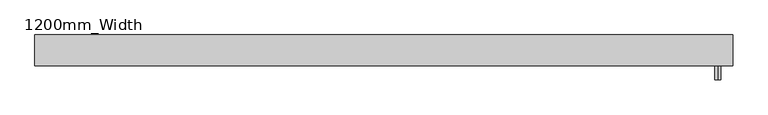
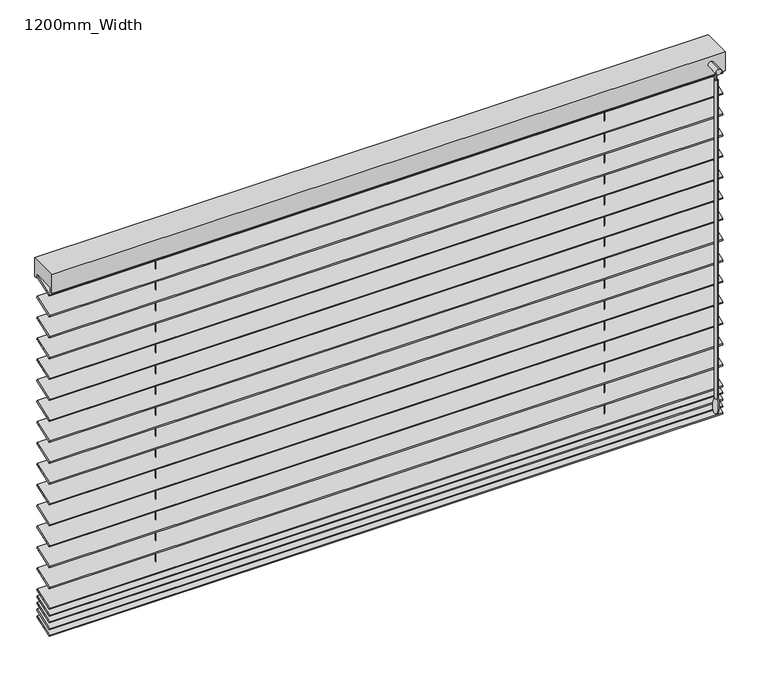
"""IFC4 building model written with IfcOpenShell, lengths in millimetres: proxy geometry, Specialty_Equipment_Venetian_Blind_Half_Down : 1200mm_Width."""

from ifc_helpers import new_model, si_unit, point, frame, frame_2d, origin, place, context, project, spatial, polyline, circle_curve, ellipse_curve, trimmed, segment, composite_curve, outline, extrude, source, transform, mapped, element, save
from ifc_brep_helpers import plane_surface, cylinder_surface, revolved_surface, advanced_brep


def proxy_1200mm_width_55fef7d2(model_context):
    return source(origin(), model_context, "Body", "SolidModel", [
        extrude(outline(polyline([(0.0, -40.0), (0.0, 0.0), (1180.0, 0.0), (1180.0, -40.0), (0.0, -40.0)])), frame((-439.5079376, 65.0532351, 1447.7279746), z_axis=(0.0, -0.3420201433256684, 0.9396926207859085), x_axis=(1.0, 0.0, 0.0)), (0.0, 0.0, 1.0), 3.0625345),
        extrude(outline(polyline([(0.0, -40.0), (0.0, 0.0), (1180.0, 0.0), (1180.0, -40.0), (0.0, -40.0)])), frame((-439.5079376, 65.0532351, 1459.9116214), z_axis=(0.0, -0.3420201433256684, 0.9396926207859085), x_axis=(1.0, 0.0, 0.0)), (0.0, 0.0, 1.0), 3.0625345),
        extrude(outline(polyline([(0.0, -40.0), (0.0, 0.0), (1180.0, 0.0), (1180.0, -40.0), (0.0, -40.0)])), frame((-439.5079376, 65.0532351, 1472.7202682), z_axis=(0.0, -0.3420201433256684, 0.9396926207859085), x_axis=(1.0, 0.0, 0.0)), (0.0, 0.0, 1.0), 3.0625345),
        extrude(outline(polyline([(0.0, -40.0), (0.0, 0.0), (1180.0, 0.0), (1180.0, -40.0), (0.0, -40.0)])), frame((-439.5079376, 65.0532351, 1484.903915), z_axis=(0.0, -0.3420201433256684, 0.9396926207859085), x_axis=(1.0, 0.0, 0.0)), (0.0, 0.0, 1.0), 3.0625345),
        extrude(outline(polyline([(0.0, -40.0), (0.0, 0.0), (1180.0, 0.0), (1180.0, -40.0), (0.0, -40.0)])), frame((-439.5079376, 65.0532351, 2040.2125618), z_axis=(0.0, -0.3420201433256684, 0.9396926207859085), x_axis=(1.0, 0.0, 0.0)), (0.0, 0.0, 1.0), 3.0625345),
        extrude(outline(polyline([(0.0, -40.0), (0.0, 0.0), (1180.0, 0.0), (1180.0, -40.0), (0.0, -40.0)])), frame((-439.5079376, 65.0532351, 2001.4625618), z_axis=(0.0, -0.3420201433256684, 0.9396926207859085), x_axis=(1.0, 0.0, 0.0)), (0.0, 0.0, 1.0), 3.0625345),
        extrude(outline(polyline([(0.0, -40.0), (0.0, 0.0), (1180.0, 0.0), (1180.0, -40.0), (0.0, -40.0)])), frame((-439.5079376, 65.0532351, 1962.7125618), z_axis=(0.0, -0.3420201433256684, 0.9396926207859085), x_axis=(1.0, 0.0, 0.0)), (0.0, 0.0, 1.0), 3.0625345),
        extrude(outline(polyline([(0.0, -40.0), (0.0, 0.0), (1180.0, 0.0), (1180.0, -40.0), (0.0, -40.0)])), frame((-439.5079376, 65.0532351, 1923.9625618), z_axis=(0.0, -0.3420201433256684, 0.9396926207859085), x_axis=(1.0, 0.0, 0.0)), (0.0, 0.0, 1.0), 3.0625345),
        extrude(outline(polyline([(0.0, -40.0), (0.0, 0.0), (1180.0, 0.0), (1180.0, -40.0), (0.0, -40.0)])), frame((-439.5079376, 65.0532351, 1885.2125618), z_axis=(0.0, -0.3420201433256684, 0.9396926207859085), x_axis=(1.0, 0.0, 0.0)), (0.0, 0.0, 1.0), 3.0625345),
        extrude(outline(polyline([(0.0, -40.0), (0.0, 0.0), (1180.0, 0.0), (1180.0, -40.0), (0.0, -40.0)])), frame((-439.5079376, 65.0532351, 1846.4625618), z_axis=(0.0, -0.3420201433256684, 0.9396926207859085), x_axis=(1.0, 0.0, 0.0)), (0.0, 0.0, 1.0), 3.0625345),
        extrude(outline(polyline([(0.0, -40.0), (0.0, 0.0), (1180.0, 0.0), (1180.0, -40.0), (0.0, -40.0)])), frame((-439.5079376, 65.0532351, 1807.7125618), z_axis=(0.0, -0.3420201433256684, 0.9396926207859085), x_axis=(1.0, 0.0, 0.0)), (0.0, 0.0, 1.0), 3.0625345),
        extrude(outline(polyline([(0.0, -40.0), (0.0, 0.0), (1180.0, 0.0), (1180.0, -40.0), (0.0, -40.0)])), frame((-439.5079376, 65.0532351, 1768.9625618), z_axis=(0.0, -0.3420201433256684, 0.9396926207859085), x_axis=(1.0, 0.0, 0.0)), (0.0, 0.0, 1.0), 3.0625345),
        extrude(outline(polyline([(0.0, -40.0), (0.0, 0.0), (1180.0, 0.0), (1180.0, -40.0), (0.0, -40.0)])), frame((-439.5079376, 65.0532351, 1730.2125618), z_axis=(0.0, -0.3420201433256684, 0.9396926207859085), x_axis=(1.0, 0.0, 0.0)), (0.0, 0.0, 1.0), 3.0625345),
        extrude(outline(polyline([(0.0, -40.0), (0.0, 0.0), (1180.0, 0.0), (1180.0, -40.0), (0.0, -40.0)])), frame((-439.5079376, 65.0532351, 1691.4625618), z_axis=(0.0, -0.3420201433256684, 0.9396926207859085), x_axis=(1.0, 0.0, 0.0)), (0.0, 0.0, 1.0), 3.0625345),
        extrude(outline(polyline([(0.0, -40.0), (0.0, 0.0), (1180.0, 0.0), (1180.0, -40.0), (0.0, -40.0)])), frame((-439.5079376, 65.0532351, 1652.7125618), z_axis=(0.0, -0.3420201433256684, 0.9396926207859085), x_axis=(1.0, 0.0, 0.0)), (0.0, 0.0, 1.0), 3.0625345),
        extrude(outline(polyline([(0.0, -40.0), (0.0, 0.0), (1180.0, 0.0), (1180.0, -40.0), (0.0, -40.0)])), frame((-439.5079376, 65.0532351, 1613.9625618), z_axis=(0.0, -0.3420201433256684, 0.9396926207859085), x_axis=(1.0, 0.0, 0.0)), (0.0, 0.0, 1.0), 3.0625345),
        extrude(outline(polyline([(0.0, -40.0), (0.0, 0.0), (1180.0, 0.0), (1180.0, -40.0), (0.0, -40.0)])), frame((-439.5079376, 65.0532351, 1575.2125618), z_axis=(0.0, -0.3420201433256684, 0.9396926207859085), x_axis=(1.0, 0.0, 0.0)), (0.0, 0.0, 1.0), 3.0625345),
        extrude(outline(polyline([(0.0, -40.0), (0.0, 0.0), (1180.0, 0.0), (1180.0, -40.0), (0.0, -40.0)])), frame((-439.5079376, 65.0532351, 1536.4625618), z_axis=(0.0, -0.3420201433256684, 0.9396926207859085), x_axis=(1.0, 0.0, 0.0)), (0.0, 0.0, 1.0), 3.0625345),
        extrude(outline(polyline([(0.0, -40.0), (0.0, 0.0), (1180.0, 0.0), (1180.0, -40.0), (0.0, -40.0)])), frame((-439.5079376, 65.0532351, 1497.7125618), z_axis=(0.0, -0.3420201433256684, 0.9396926207859085), x_axis=(1.0, 0.0, 0.0)), (0.0, 0.0, 1.0), 3.0625345),
        extrude(outline(polyline([(0.0, -40.0), (0.0, 0.0), (1180.0, 0.0), (1180.0, -40.0), (0.0, -40.0)])), frame((-439.5079376, 65.0532351, 2078.9625618), z_axis=(0.0, -0.3420201433256684, 0.9396926207859085), x_axis=(1.0, 0.0, 0.0)), (0.0, 0.0, 1.0), 3.0625345),
        extrude(outline(composite_curve([segment(trimmed(circle_curve(frame_2d((-242.8412709, 45.2119342)), 0.5), [point((-243.3412709, 45.2119342))], [point((-242.3412709, 45.2119342))], False, "CARTESIAN"), True, "CONTINUOUS"), segment(trimmed(circle_curve(frame_2d((-242.8412709, 45.2119342)), 0.5), [point((-242.3412709, 45.2119342))], [point((-243.3412709, 45.2119342))], False, "CARTESIAN"), True, "CONTINUOUS")], self_intersect=False)), frame((0.0, 0.0, 1434.9736305), z_axis=(0.0, 0.0, 1.0), x_axis=(1.0, 0.0, 0.0)), (0.0, 0.0, 1.0), 648.2712578),
        extrude(outline(composite_curve([segment(trimmed(circle_curve(frame_2d((543.8253958, 45.2119342)), 0.5), [point((543.3253958, 45.2119342))], [point((544.3253958, 45.2119342))], False, "CARTESIAN"), True, "CONTINUOUS"), segment(trimmed(circle_curve(frame_2d((543.8253958, 45.2119342)), 0.5), [point((544.3253958, 45.2119342))], [point((543.3253958, 45.2119342))], False, "CARTESIAN"), True, "CONTINUOUS")], self_intersect=False)), frame((0.0, 0.0, 1434.9736305), z_axis=(0.0, 0.0, 1.0), x_axis=(1.0, 0.0, 0.0)), (0.0, 0.0, 1.0), 648.2712578),
        advanced_brep(
        [(715.4920624, 4.7248495, 2091.3243671), (715.4920624, 2.7248495, 2091.3243671), (715.4920624, 3.7248495, 2091.3243671), (715.4920624, 4.7248495, 2076.3243671), (715.4920624, 2.7248495, 2076.3243671), (715.4920624, 6.7248495, 2076.3243671), (715.4920624, 0.7248495, 2076.3243671), (715.4920624, 6.7248495, 1486.909931), (715.4920624, 0.7248495, 1486.909931), (715.4920624, 7.2513368, 1460.0), (715.4920624, 0.1983622, 1460.0), (715.4920624, 3.7248495, 1460.0)],
        [
            (0, 1, circle_curve(frame((715.4920624, 3.7248495, 2091.3243671), z_axis=(0.0, 0.0, 1.0), x_axis=(0.0, -1.0, 0.0)), 1.0)),
            (1, 2),
            (2, 0),
            (1, 0, circle_curve(frame((715.4920624, 3.7248495, 2091.3243671), z_axis=(0.0, 0.0, 1.0), x_axis=(0.0, -1.0, 0.0)), 1.0)),
            (3, 4, circle_curve(frame((715.4920624, 3.7248495, 2076.3243671), z_axis=(0.0, 0.0, 1.0), x_axis=(0.0, -1.0, 0.0)), 1.0)),
            (4, 1),
            (0, 3),
            (4, 3, circle_curve(frame((715.4920624, 3.7248495, 2076.3243671), z_axis=(0.0, 0.0, 1.0), x_axis=(0.0, -1.0, 0.0)), 1.0)),
            (5, 6, circle_curve(frame((715.4920624, 3.7248495, 2076.3243671), z_axis=(0.0, 0.0, 1.0), x_axis=(0.0, -1.0, 0.0)), 3.0)),
            (6, 4),
            (3, 5),
            (6, 5, circle_curve(frame((715.4920624, 3.7248495, 2076.3243671), z_axis=(0.0, 0.0, 1.0), x_axis=(0.0, -1.0, 0.0)), 3.0)),
            (7, 8, circle_curve(frame((715.4920624, 3.7248495, 1486.909931), z_axis=(0.0, 0.0, 1.0), x_axis=(0.0, -1.0, 0.0)), 3.0)),
            (8, 6),
            (5, 7),
            (8, 7, circle_curve(frame((715.4920624, 3.7248495, 1486.909931), z_axis=(0.0, 0.0, 1.0), x_axis=(0.0, -1.0, 0.0)), 3.0)),
            (9, 10, circle_curve(frame((715.4920624, 3.7248495, 1460.0), z_axis=(0.0, 0.0, 1.0), x_axis=(0.0, -1.0, 0.0)), 3.5264873)),
            (10, 8, circle_curve(frame((715.4920624, 49.2720063, 1472.5), z_axis=(-1.0, 0.0, 0.0), x_axis=(0.0, 1.0, 0.0)), 50.6406214)),
            (7, 9, circle_curve(frame((715.4920624, -41.8223072, 1472.5), z_axis=(-1.0, 0.0, 0.0), x_axis=(0.0, -1.0, 0.0)), 50.6406214)),
            (10, 9, circle_curve(frame((715.4920624, 3.7248495, 1460.0), z_axis=(0.0, 0.0, 1.0), x_axis=(0.0, -1.0, 0.0)), 3.5264873)),
            (11, 10),
            (9, 11),
        ],
        [
            plane_surface(frame((715.4920624, 3.7248495, 2091.3243671), z_axis=(0.0, 0.0, 1.0), x_axis=(0.0, -1.0, 0.0))),
            cylinder_surface(frame((715.4920624, 3.7248495, 1191.3243671), z_axis=(0.0, 0.0, -1.0), x_axis=(0.0, -1.0, 0.0)), 1.0),
            plane_surface(frame((715.4920624, 3.7248495, 2076.3243671), z_axis=(0.0, 0.0, 1.0), x_axis=(0.0, -1.0, 0.0))),
            cylinder_surface(frame((715.4920624, 3.7248495, 1191.3243671), z_axis=(0.0, 0.0, -1.0), x_axis=(0.0, -1.0, 0.0)), 3.0),
            revolved_surface(trimmed(ellipse_curve(frame((715.4920624, 49.2720063, 1472.5), z_axis=(1.0, 0.0, 0.0), x_axis=(0.0, 1.0, 0.0)), 50.6406214, 50.6406214), [point((715.4920624, 0.7248495, 1486.909931))], [point((715.4920624, 0.1983622, 1460.0))], True, "CARTESIAN"), (715.4920624, 3.7248495, 1191.3243671), (0.0, 0.0, -1.0)),
            plane_surface(frame((715.4920624, 3.7248495, 1460.0), z_axis=(0.0, 0.0, -1.0), x_axis=(0.0, -1.0, 0.0))),
        ],
        [
            (0, [[1, 2, 3]]),
            (0, [[4, -3, -2]]),
            (1, [[5, 6, -1, 7]]),
            (1, [[8, -7, -4, -6]]),
            (2, [[9, 10, -5, 11]]),
            (2, [[12, -11, -8, -10]]),
            (3, [[13, 14, -9, 15]]),
            (3, [[16, -15, -12, -14]]),
            (4, [[17, 18, -13, 19]]),
            (4, [[20, -19, -16, -18]]),
            (5, [[21, -17, 22]]),
            (5, [[-22, -20, -21]]),
        ],
    ),
        extrude(outline(composite_curve([segment(trimmed(circle_curve(frame_2d((2095.9171213, 715.4920624)), 5.0), [point((2100.9171213, 715.4920624))], [point((2090.9171213, 715.4920624))], False, "CARTESIAN"), True, "CONTINUOUS"), segment(trimmed(circle_curve(frame_2d((2095.9171213, 715.4920624)), 5.0), [point((2090.9171213, 715.4920624))], [point((2100.9171213, 715.4920624))], False, "CARTESIAN"), True, "CONTINUOUS")], self_intersect=False)), frame((0.0, -4.4512463, 0.0), z_axis=(0.0, 1.0, 0.0), x_axis=(0.0, 0.0, 1.0)), (0.0, 0.0, 1.0), 23.7809602),
        extrude(outline(polyline([(19.329714, 2110.0), (71.0941545, 2110.0), (71.0941545, 2075.0), (66.0941545, 2075.0), (66.0941545, 2083.2448883), (24.329714, 2083.2448883), (24.329714, 2075.0), (19.329714, 2075.0), (19.329714, 2110.0)])), frame((-439.5079376, 0.0, 0.0), z_axis=(1.0, 0.0, 0.0), x_axis=(0.0, 1.0, 0.0)), (0.0, 0.0, 1.0), 1180.0),
    ])


if __name__ == "__main__":
    model = new_model("IFC4")
    model_context = context("Model", 3, world=origin())
    ifc_project = project(units=[si_unit("LENGTHUNIT", "METRE", prefix="MILLI")], contexts=[model_context])
    site = spatial("IfcSite", under=ifc_project)
    building = spatial("IfcBuilding", under=site)
    placement = place(None, origin())
    proxy_1200mm_width_shape = proxy_1200mm_width_55fef7d2(model_context)
    element("IfcBuildingElementProxy", 1, Name="Specialty_Equipment_Venetian_Blind_Half_Down : 1200mm_Width", ObjectType="Specialty_Equipment_Venetian_Blind_Half_Down : 1200mm_Width", at=placement, inside=building, context=model_context, shape_type="MappedRepresentation", body=[
        mapped(proxy_1200mm_width_shape, transform((0.0, 0.0, 0.0), x_axis=(1.0, 0.0, 0.0), y_axis=(0.0, 1.0, 0.0), z_axis=(0.0, 0.0, 1.0))),
    ])
    save(model, "model.ifc")

# Revit data of these elements
# Type "Specialty_Equipment_Venetian_Blind_Half_Down : 1200mm_Width"
#   Keynote = "N10/240"
#   Opening Width = 1200 mm
#   End Offset = 10 mm
#   Blind Length = 1180 mm
#   Blind Fixing Height = 2110 mm
#   Blind Depth = 980 mm
#   Blind Angle = 20.00°
#   Blade Depth = 40 mm
#   No of Blades = 25
#   Material Blind = Wood - Birch
#   Default Elevation = 0
# Element 1 (IfcBuildingElementProxy, "Specialty_Equipment_Venetian_Blind_Half_Down : 1200mm_Width")
#   Materials on its faces: "Wood - Birch"
# Materials
#   "Wood - Birch": class "Wood", colour RGB 224 178 126, transparency 0
